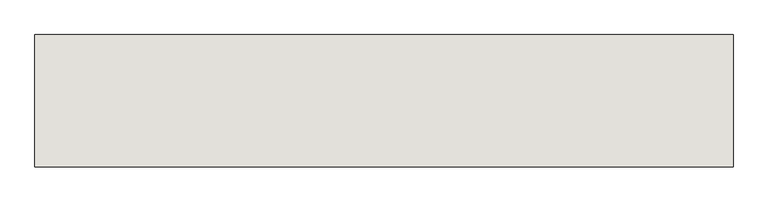
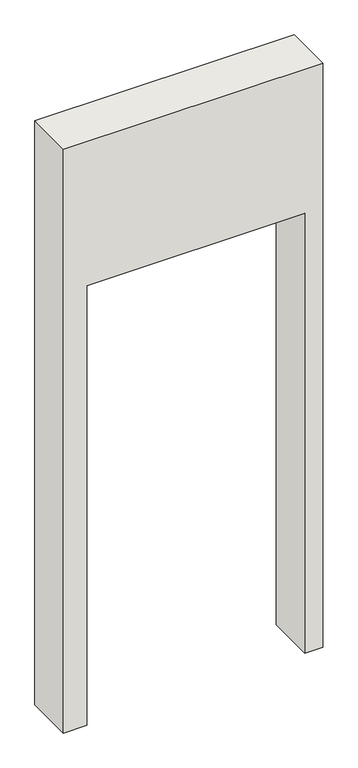
"""IFC4 building model written with IfcOpenShell, lengths in millimetres: wall geometry, Holzwand."""

from ifc_helpers import new_model, si_unit, frame, origin, place, context, project, spatial, polyline, outline, extrude, source, transform, mapped, element, save


def wall_c629b92f(model_context):
    return source(origin(), model_context, "Body", "SweptSolid", [
        extrude(outline(polyline([(1890.0, 980.7436213), (0.0, 980.7436213), (0.0, 1055.0), (2510.0, 1055.0), (2510.0, 0.0), (0.0, 0.0), (0.0, 95.7436213), (1890.0, 95.7436213), (1890.0, 980.7436213)])), frame((0.0, 0.0, 0.0), z_axis=(0.0, 1.0, 0.0), x_axis=(0.0, 0.0, 1.0)), (0.0, 0.0, 1.0), 200.0),
    ])


if __name__ == "__main__":
    model = new_model("IFC4")
    model_context = context("Model", 3, world=origin())
    ifc_project = project(units=[si_unit("LENGTHUNIT", "METRE", prefix="MILLI")], contexts=[model_context])
    site = spatial("IfcSite", under=ifc_project)
    building = spatial("IfcBuilding", under=site)
    placement = place(None, origin())
    wall_shape = wall_c629b92f(model_context)
    element("IfcWall", 1, ObjectType="Holzwand", at=placement, inside=building, context=model_context, shape_type="MappedRepresentation", body=[
        mapped(wall_shape, transform((0.0, 0.0, 0.0), x_axis=(1.0, 0.0, 0.0), y_axis=(0.0, 1.0, 0.0), z_axis=(0.0, 0.0, 1.0))),
    ])
    save(model, "model.ifc")

# Revit data of these elements
# Element 1 (IfcWall, "Holzwand")
#   Materials on its faces: "holzschalung"
# Materials
#   "holzschalung": class "Unassigned", colour RGB 128 128 128, transparency 0
